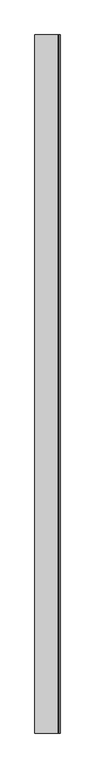
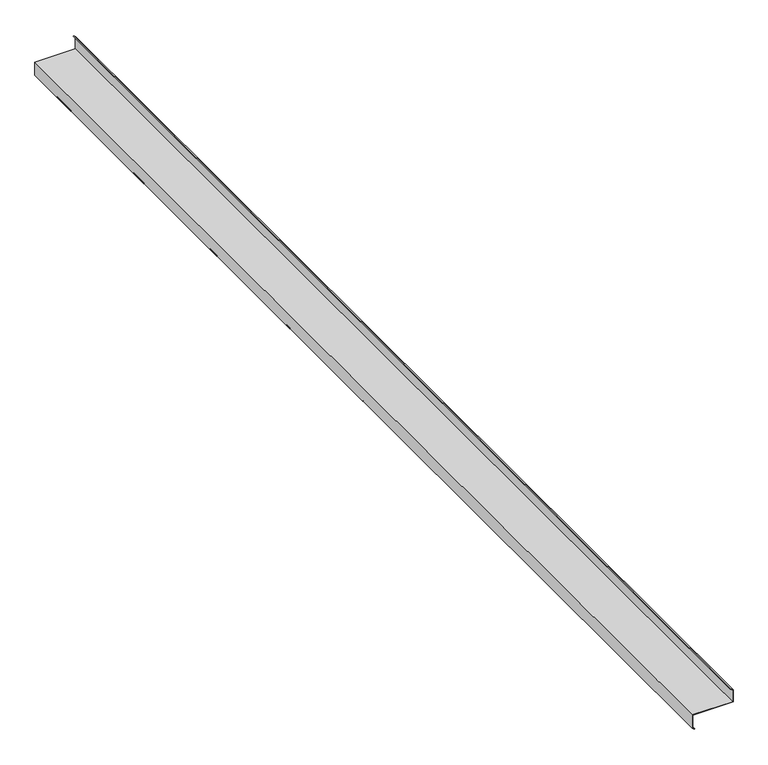
"""IFC4 building model written with IfcOpenShell, lengths in millimetres: proxy geometry, Generic Models 7:Generic Models 1:1:Generic Models 1:1 : Generic Models 7:Generic Models 1:337419:34 : Generic Models 7:Generic Models 1:1:Generic Models 1:1 : Generic Models 7:Generic Models 1:337419:306201."""

from ifc_helpers import new_model, si_unit, frame, origin, place, context, project, spatial, polyline, outline, extrude, source, transform, mapped, element, save


def generic_models_fae29493(model_context):
    return source(origin(), model_context, "Body", "SweptSolid", [
        extrude(outline(polyline([(1396.3591063, 667530.7466425), (1384.7904762, 667544.533599), (1309.4890623, 667544.533599), (1309.4890623, 667293.3117239), (1223.7640623, 667293.3117239), (1211.5189583, 667307.9048706), (1213.6471255, 667309.6906149), (1225.0595233, 667296.0898489), (1306.7109373, 667296.0898489), (1306.7109373, 667547.3117239), (1386.0859372, 667547.3117239), (1398.3310411, 667532.7185773), (1396.3591063, 667530.7466425)])), frame((0.0, -571669.6163841, 0.0), z_axis=(0.0, 1.0, 0.0), x_axis=(0.0, 0.0, 1.0)), (0.0, 0.0, 1.0), 7061.2),
    ])


if __name__ == "__main__":
    model = new_model("IFC4")
    model_context = context("Model", 3, world=origin())
    ifc_project = project(units=[si_unit("LENGTHUNIT", "METRE", prefix="MILLI")], contexts=[model_context])
    site = spatial("IfcSite", under=ifc_project)
    building = spatial("IfcBuilding", under=site)
    placement = place(None, origin())
    generic_models_shape = generic_models_fae29493(model_context)
    element("IfcBuildingElementProxy", 1, Name="Generic Models 7:Generic Models 1:1:Generic Models 1:1 : Generic Models 7:Generic Models 1:337419:34 : Generic Models 7:Generic Models 1:1:Generic Models 1:1 : Generic Models 7:Generic Models 1:337419:306201", ObjectType="Generic Models 7:Generic Models 1:1:Generic Models 1:1 : Generic Models 7:Generic Models 1:337419:34 : Generic Models 7:Generic Models 1:1:Generic Models 1:1 : Generic Models 7:Generic Models 1:337419:306201", at=placement, inside=building, context=model_context, shape_type="MappedRepresentation", body=[
        mapped(generic_models_shape, transform((0.0, 0.0, 0.0), x_axis=(1.0, 0.0, 0.0), y_axis=(0.0, 1.0, 0.0), z_axis=(0.0, 0.0, 1.0))),
    ])
    save(model, "model.ifc")

# Revit data of these elements
# Type "Generic Models 7:Generic Models 1:1:Generic Models 1:1 : Generic Models 7:Generic Models 1:337419:34 : Generic Models 7:Generic Models 1:1:Generic Models 1:1 : Generic Models 7:Generic Models 1:337419:306201"
#   NameOverride = "Generic Models 7:Generic Models 1:1:Generic Models 1:1 : Generic Models 7:Generic Models 1:337419:306201"
#   ObjectTypeOverride = "Generic Models 1:1 : Generic Models 7:Generic Models 1:337419"
#   Reference = "Generic Models 1"
#   Tag = "306201"
# Element 1 (IfcBuildingElementProxy, "Generic Models 7:Generic Models 1:1:Generic Models 1:1 : Generic Models 7:Generic Models 1:337419:34 : Generic Models 7:Generic Models 1:1:Generic Models 1:1 : Generic Models 7:Generic Models 1:337419:306201")
#   Materials on its faces: "CEE' SECTION (8.0x3.5C - SEE STRUCT. DWGS)"
# Materials
#   "CEE' SECTION (8.0x3.5C - SEE STRUCT. DWGS)": class "Unassigned", colour RGB 210 209 208, transparency 0, Keynote = "M05121300.02", Cost = 0
